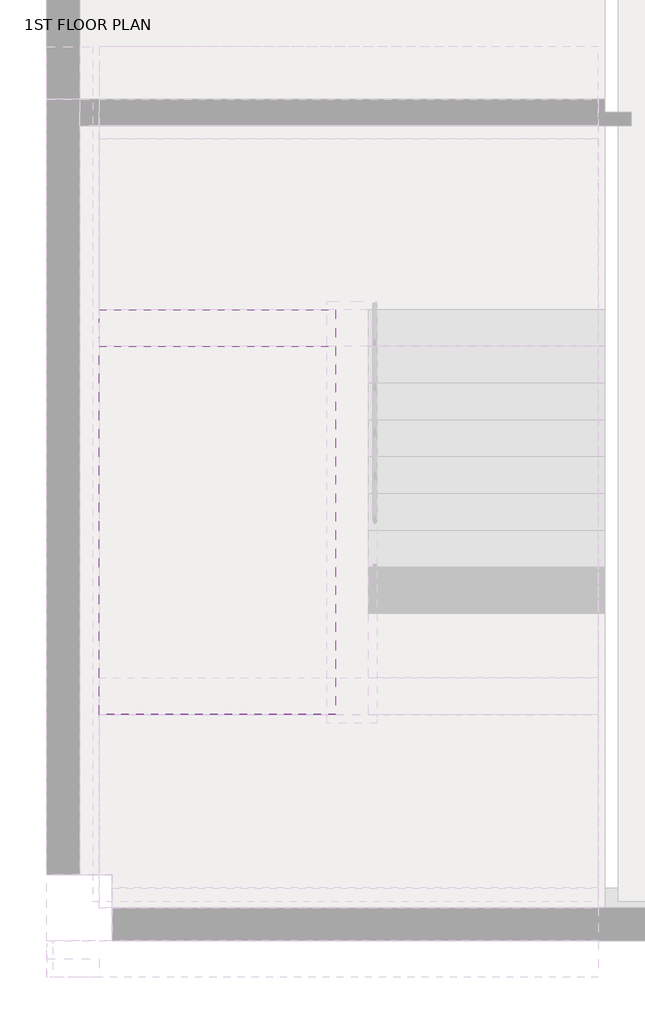
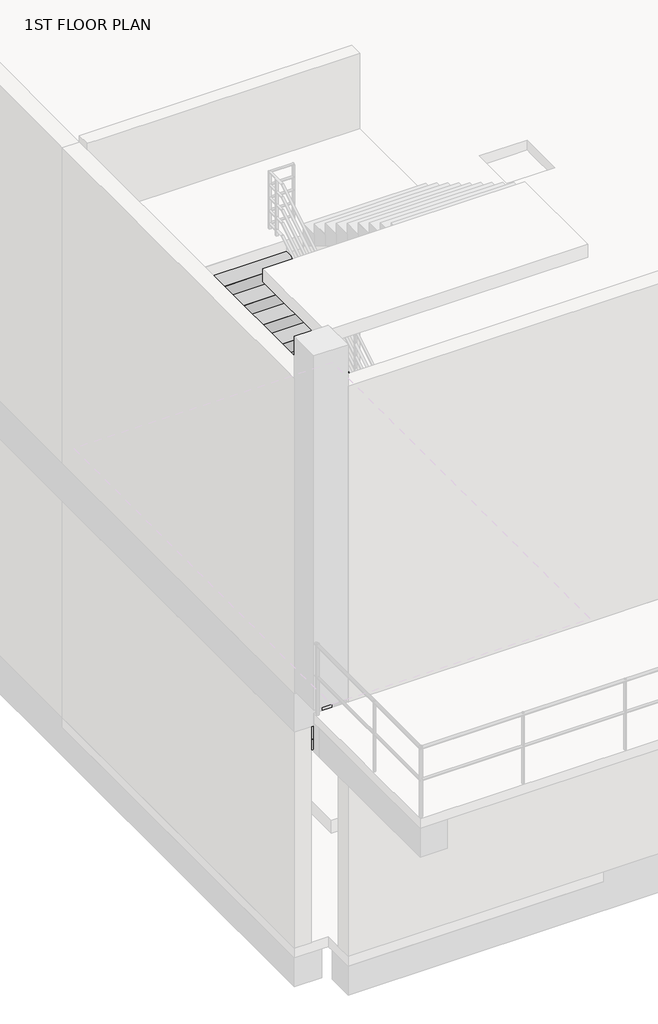
# One storey, part 6 of 9: 2 stair flights.
"""IFC4 building model written with IfcOpenShell, lengths in millimetres."""

from ifc_helpers import new_model, si_unit, frame, origin, place, context, project, spatial, polyline, outline, extrude, faceted_brep, element, save

model = new_model("IFC4")

# Units and contexts
model_context = context("Model", 3, world=origin())
ifc_project = project(units=[si_unit("LENGTHUNIT", "METRE", prefix="MILLI")], contexts=[model_context])

# Site, building, storey
site = spatial("IfcSite", under=ifc_project)
building = spatial("IfcBuilding", under=site)
storey = spatial("IfcBuildingStorey", under=building, Name="1ST FLOOR PLAN", Elevation=600.005241)

# Stair flights
placement = place(None, origin())
element("IfcStairFlight", 1, ObjectType="1mm 디딤판", at=placement, inside=storey, context=model_context, shape_type="SolidModel", body=[
    faceted_brep([(50.0, 22699.5208589, 2765.8781576), (50.0, 22419.5208589, 2765.8781576), (1850.0, 22419.5208589, 2765.8781576), (1850.0, 22699.5208589, 2765.8781576), (50.0, 22699.5208589, 2591.3160232), (50.0, 22419.5208589, 2424.6493565), (50.0, 22419.5208589, 2599.211491), (1850.0, 22419.5208589, 2424.6493565), (1850.0, 22699.5208589, 2591.3160232), (50.0, 22979.5208589, 2932.5448243), (50.0, 22699.5208589, 2932.5448243), (1850.0, 22699.5208589, 2932.5448243), (1850.0, 22979.5208589, 2932.5448243), (50.0, 22979.5208589, 2757.9826899), (1850.0, 22979.5208589, 2757.9826899), (50.0, 23259.5208589, 3099.211491), (50.0, 22979.5208589, 3099.211491), (1850.0, 22979.5208589, 3099.211491), (1850.0, 23259.5208589, 3099.211491), (50.0, 23259.5208589, 2924.6493565), (1850.0, 23259.5208589, 2924.6493565), (50.0, 23539.5208589, 3265.8781576), (50.0, 23259.5208589, 3265.8781576), (1850.0, 23259.5208589, 3265.8781576), (1850.0, 23539.5208589, 3265.8781576), (50.0, 23539.5208589, 3091.3160232), (1850.0, 23539.5208589, 3091.3160232), (50.0, 23819.5208589, 3432.5448243), (50.0, 23539.5208589, 3432.5448243), (1850.0, 23539.5208589, 3432.5448243), (1850.0, 23819.5208589, 3432.5448243), (50.0, 23819.5208589, 3257.9826899), (1850.0, 23819.5208589, 3257.9826899), (50.0, 24099.5208589, 3599.211491), (50.0, 23819.5208589, 3599.211491), (1850.0, 23819.5208589, 3599.211491), (1850.0, 24099.5208589, 3599.211491), (50.0, 24099.5208589, 3424.6493565), (1850.0, 24099.5208589, 3424.6493565), (50.0, 24379.5208589, 3765.8781576), (50.0, 24099.5208589, 3765.8781576), (1850.0, 24099.5208589, 3765.8781576), (1850.0, 24379.5208589, 3765.8781576), (50.0, 24379.5208589, 3591.3160232), (1850.0, 24379.5208589, 3591.3160232), (50.0, 24659.5208589, 3932.5448243), (50.0, 24379.5208589, 3932.5448243), (1850.0, 24379.5208589, 3932.5448243), (1850.0, 24659.5208589, 3932.5448243), (50.0, 24659.5208589, 3757.9826899), (1850.0, 24659.5208589, 3757.9826899), (50.0, 24939.5208589, 4099.211491), (50.0, 24659.5208589, 4099.211491), (1850.0, 24659.5208589, 4099.211491), (1850.0, 24939.5208589, 4099.211491), (50.0, 24939.5208589, 3924.6493565), (1850.0, 24939.5208589, 3924.6493565), (50.0, 25219.5208589, 4265.8781576), (50.0, 24939.5208589, 4265.8781576), (1850.0, 24939.5208589, 4265.8781576), (1850.0, 25219.5208589, 4265.8781576), (50.0, 25219.5208589, 4091.3160232), (1850.0, 25219.5208589, 4091.3160232), (50.0, 25499.5208589, 4432.5448243), (50.0, 25219.5208589, 4432.5448243), (1850.0, 25219.5208589, 4432.5448243), (1850.0, 25499.5208589, 4432.5448243), (50.0, 25499.5208589, 4257.9826899), (1850.0, 25499.5208589, 4257.9826899), (1850.0, 25499.5208589, 4399.211491)], [[[0, 1, 2, 3]], [[1, 0, 4, 5, 6]], [[2, 1, 6, 5, 7]], [[3, 2, 7, 8]], [[9, 10, 11, 12]], [[10, 9, 13, 4, 0]], [[11, 10, 0, 3]], [[12, 11, 3, 8, 14]], [[15, 16, 17, 18]], [[16, 15, 19, 13, 9]], [[17, 16, 9, 12]], [[18, 17, 12, 14, 20]], [[21, 22, 23, 24]], [[22, 21, 25, 19, 15]], [[23, 22, 15, 18]], [[24, 23, 18, 20, 26]], [[27, 28, 29, 30]], [[28, 27, 31, 25, 21]], [[29, 28, 21, 24]], [[30, 29, 24, 26, 32]], [[33, 34, 35, 36]], [[34, 33, 37, 31, 27]], [[35, 34, 27, 30]], [[36, 35, 30, 32, 38]], [[39, 40, 41, 42]], [[40, 39, 43, 37, 33]], [[41, 40, 33, 36]], [[42, 41, 36, 38, 44]], [[45, 46, 47, 48]], [[46, 45, 49, 43, 39]], [[47, 46, 39, 42]], [[48, 47, 42, 44, 50]], [[51, 52, 53, 54]], [[52, 51, 55, 49, 45]], [[53, 52, 45, 48]], [[54, 53, 48, 50, 56]], [[57, 58, 59, 60]], [[58, 57, 61, 55, 51]], [[59, 58, 51, 54]], [[60, 59, 54, 56, 62]], [[63, 64, 65, 66]], [[64, 63, 67, 61, 57]], [[65, 64, 57, 60]], [[66, 65, 60, 62, 68, 69]], [[63, 66, 69, 68, 67]], [[5, 4, 13, 19, 25, 31, 37, 43, 49, 55, 61, 67, 68, 62, 56, 50, 44, 38, 32, 26, 20, 14, 8, 7]]]),
    extrude(outline(polyline([(50.0, 22699.5208589), (1850.0, 22699.5208589), (1850.0, 22419.5208589), (50.0, 22419.5208589), (50.0, 22699.5208589)])), frame((0.0, 0.0, 2765.8781576), z_axis=(0.0, 0.0, 1.0), x_axis=(1.0, 0.0, 0.0)), (0.0, 0.0, 1.0), 0.79375),
    extrude(outline(polyline([(50.0, 22979.5208589), (1850.0, 22979.5208589), (1850.0, 22699.5208589), (50.0, 22699.5208589), (50.0, 22979.5208589)])), frame((0.0, 0.0, 2932.5448243), z_axis=(0.0, 0.0, 1.0), x_axis=(1.0, 0.0, 0.0)), (0.0, 0.0, 1.0), 0.79375),
    extrude(outline(polyline([(50.0, 23259.5208589), (1850.0, 23259.5208589), (1850.0, 22979.5208589), (50.0, 22979.5208589), (50.0, 23259.5208589)])), frame((0.0, 0.0, 3099.211491), z_axis=(0.0, 0.0, 1.0), x_axis=(1.0, 0.0, 0.0)), (0.0, 0.0, 1.0), 0.79375),
    extrude(outline(polyline([(50.0, 23539.5208589), (1850.0, 23539.5208589), (1850.0, 23259.5208589), (50.0, 23259.5208589), (50.0, 23539.5208589)])), frame((0.0, 0.0, 3265.8781576), z_axis=(0.0, 0.0, 1.0), x_axis=(1.0, 0.0, 0.0)), (0.0, 0.0, 1.0), 0.79375),
    extrude(outline(polyline([(50.0, 23819.5208589), (1850.0, 23819.5208589), (1850.0, 23539.5208589), (50.0, 23539.5208589), (50.0, 23819.5208589)])), frame((0.0, 0.0, 3432.5448243), z_axis=(0.0, 0.0, 1.0), x_axis=(1.0, 0.0, 0.0)), (0.0, 0.0, 1.0), 0.79375),
    extrude(outline(polyline([(50.0, 24099.5208589), (1850.0, 24099.5208589), (1850.0, 23819.5208589), (50.0, 23819.5208589), (50.0, 24099.5208589)])), frame((0.0, 0.0, 3599.211491), z_axis=(0.0, 0.0, 1.0), x_axis=(1.0, 0.0, 0.0)), (0.0, 0.0, 1.0), 0.79375),
    extrude(outline(polyline([(50.0, 24379.5208589), (1850.0, 24379.5208589), (1850.0, 24099.5208589), (50.0, 24099.5208589), (50.0, 24379.5208589)])), frame((0.0, 0.0, 3765.8781576), z_axis=(0.0, 0.0, 1.0), x_axis=(1.0, 0.0, 0.0)), (0.0, 0.0, 1.0), 0.79375),
    extrude(outline(polyline([(50.0, 24659.5208589), (1850.0, 24659.5208589), (1850.0, 24379.5208589), (50.0, 24379.5208589), (50.0, 24659.5208589)])), frame((0.0, 0.0, 3932.5448243), z_axis=(0.0, 0.0, 1.0), x_axis=(1.0, 0.0, 0.0)), (0.0, 0.0, 1.0), 0.79375),
    extrude(outline(polyline([(50.0, 24939.5208589), (1850.0, 24939.5208589), (1850.0, 24659.5208589), (50.0, 24659.5208589), (50.0, 24939.5208589)])), frame((0.0, 0.0, 4099.211491), z_axis=(0.0, 0.0, 1.0), x_axis=(1.0, 0.0, 0.0)), (0.0, 0.0, 1.0), 0.79375),
    extrude(outline(polyline([(50.0, 25219.5208589), (1850.0, 25219.5208589), (1850.0, 24939.5208589), (50.0, 24939.5208589), (50.0, 25219.5208589)])), frame((0.0, 0.0, 4265.8781576), z_axis=(0.0, 0.0, 1.0), x_axis=(1.0, 0.0, 0.0)), (0.0, 0.0, 1.0), 0.79375),
    extrude(outline(polyline([(50.0, 25499.5208589), (1850.0, 25499.5208589), (1850.0, 25219.5208589), (50.0, 25219.5208589), (50.0, 25499.5208589)])), frame((0.0, 0.0, 4432.5448243), z_axis=(0.0, 0.0, 1.0), x_axis=(1.0, 0.0, 0.0)), (0.0, 0.0, 1.0), 0.79375),
])
element("IfcStairFlight", 2, ObjectType="1mm 디딤판", at=placement, inside=storey, context=model_context, shape_type="SolidModel", body=[
    faceted_brep([(50.0, 22699.5208589, 6661.711491), (50.0, 22419.5208589, 6661.711491), (1850.0, 22419.5208589, 6661.711491), (1850.0, 22699.5208589, 6661.711491), (50.0, 22699.5208589, 6485.7058943), (50.0, 22419.5208589, 6313.8308943), (50.0, 22419.5208589, 6489.836491), (1850.0, 22419.5208589, 6313.8308943), (1850.0, 22699.5208589, 6485.7058943), (50.0, 22979.5208589, 6833.586491), (50.0, 22699.5208589, 6833.586491), (1850.0, 22699.5208589, 6833.586491), (1850.0, 22979.5208589, 6833.586491), (50.0, 22979.5208589, 6657.5808943), (1850.0, 22979.5208589, 6657.5808943), (50.0, 23259.5208589, 7005.461491), (50.0, 22979.5208589, 7005.461491), (1850.0, 22979.5208589, 7005.461491), (1850.0, 23259.5208589, 7005.461491), (50.0, 23259.5208589, 6829.4558943), (1850.0, 23259.5208589, 6829.4558943), (50.0, 23539.5208589, 7177.336491), (50.0, 23259.5208589, 7177.336491), (1850.0, 23259.5208589, 7177.336491), (1850.0, 23539.5208589, 7177.336491), (50.0, 23539.5208589, 7001.3308943), (1850.0, 23539.5208589, 7001.3308943), (50.0, 23819.5208589, 7349.211491), (50.0, 23539.5208589, 7349.211491), (1850.0, 23539.5208589, 7349.211491), (1850.0, 23819.5208589, 7349.211491), (50.0, 23819.5208589, 7173.2058943), (1850.0, 23819.5208589, 7173.2058943), (50.0, 24099.5208589, 7521.086491), (50.0, 23819.5208589, 7521.086491), (1850.0, 23819.5208589, 7521.086491), (1850.0, 24099.5208589, 7521.086491), (50.0, 24099.5208589, 7345.0808943), (1850.0, 24099.5208589, 7345.0808943), (50.0, 24379.5208589, 7692.961491), (50.0, 24099.5208589, 7692.961491), (1850.0, 24099.5208589, 7692.961491), (1850.0, 24379.5208589, 7692.961491), (50.0, 24379.5208589, 7516.9558943), (1850.0, 24379.5208589, 7516.9558943), (50.0, 24659.5208589, 7864.836491), (50.0, 24379.5208589, 7864.836491), (1850.0, 24379.5208589, 7864.836491), (1850.0, 24659.5208589, 7864.836491), (50.0, 24659.5208589, 7688.8308943), (1850.0, 24659.5208589, 7688.8308943), (50.0, 24939.5208589, 8036.711491), (50.0, 24659.5208589, 8036.711491), (1850.0, 24659.5208589, 8036.711491), (1850.0, 24939.5208589, 8036.711491), (50.0, 24939.5208589, 7860.7058943), (1850.0, 24939.5208589, 7860.7058943), (50.0, 25219.5208589, 8208.586491), (50.0, 24939.5208589, 8208.586491), (1850.0, 24939.5208589, 8208.586491), (1850.0, 25219.5208589, 8208.586491), (50.0, 25219.5208589, 8032.5808943), (1850.0, 25219.5208589, 8032.5808943), (1850.0, 25219.5208589, 8180.461491)], [[[0, 1, 2, 3]], [[1, 0, 4, 5, 6]], [[2, 1, 6, 5, 7]], [[3, 2, 7, 8]], [[9, 10, 11, 12]], [[10, 9, 13, 4, 0]], [[11, 10, 0, 3]], [[12, 11, 3, 8, 14]], [[15, 16, 17, 18]], [[16, 15, 19, 13, 9]], [[17, 16, 9, 12]], [[18, 17, 12, 14, 20]], [[21, 22, 23, 24]], [[22, 21, 25, 19, 15]], [[23, 22, 15, 18]], [[24, 23, 18, 20, 26]], [[27, 28, 29, 30]], [[28, 27, 31, 25, 21]], [[29, 28, 21, 24]], [[30, 29, 24, 26, 32]], [[33, 34, 35, 36]], [[34, 33, 37, 31, 27]], [[35, 34, 27, 30]], [[36, 35, 30, 32, 38]], [[39, 40, 41, 42]], [[40, 39, 43, 37, 33]], [[41, 40, 33, 36]], [[42, 41, 36, 38, 44]], [[45, 46, 47, 48]], [[46, 45, 49, 43, 39]], [[47, 46, 39, 42]], [[48, 47, 42, 44, 50]], [[51, 52, 53, 54]], [[52, 51, 55, 49, 45]], [[53, 52, 45, 48]], [[54, 53, 48, 50, 56]], [[57, 58, 59, 60]], [[58, 57, 61, 55, 51]], [[59, 58, 51, 54]], [[60, 59, 54, 56, 62, 63]], [[57, 60, 63, 62, 61]], [[5, 4, 13, 19, 25, 31, 37, 43, 49, 55, 61, 62, 56, 50, 44, 38, 32, 26, 20, 14, 8, 7]]]),
    extrude(outline(polyline([(50.0, 22699.5208589), (1850.0, 22699.5208589), (1850.0, 22419.5208589), (50.0, 22419.5208589), (50.0, 22699.5208589)])), frame((0.0, 0.0, 6661.711491), z_axis=(0.0, 0.0, 1.0), x_axis=(1.0, 0.0, 0.0)), (0.0, 0.0, 1.0), 0.79375),
    extrude(outline(polyline([(50.0, 22979.5208589), (1850.0, 22979.5208589), (1850.0, 22699.5208589), (50.0, 22699.5208589), (50.0, 22979.5208589)])), frame((0.0, 0.0, 6833.586491), z_axis=(0.0, 0.0, 1.0), x_axis=(1.0, 0.0, 0.0)), (0.0, 0.0, 1.0), 0.79375),
    extrude(outline(polyline([(50.0, 23259.5208589), (1850.0, 23259.5208589), (1850.0, 22979.5208589), (50.0, 22979.5208589), (50.0, 23259.5208589)])), frame((0.0, 0.0, 7005.461491), z_axis=(0.0, 0.0, 1.0), x_axis=(1.0, 0.0, 0.0)), (0.0, 0.0, 1.0), 0.79375),
    extrude(outline(polyline([(50.0, 23539.5208589), (1850.0, 23539.5208589), (1850.0, 23259.5208589), (50.0, 23259.5208589), (50.0, 23539.5208589)])), frame((0.0, 0.0, 7177.336491), z_axis=(0.0, 0.0, 1.0), x_axis=(1.0, 0.0, 0.0)), (0.0, 0.0, 1.0), 0.79375),
    extrude(outline(polyline([(50.0, 23819.5208589), (1850.0, 23819.5208589), (1850.0, 23539.5208589), (50.0, 23539.5208589), (50.0, 23819.5208589)])), frame((0.0, 0.0, 7349.211491), z_axis=(0.0, 0.0, 1.0), x_axis=(1.0, 0.0, 0.0)), (0.0, 0.0, 1.0), 0.79375),
    extrude(outline(polyline([(50.0, 24099.5208589), (1850.0, 24099.5208589), (1850.0, 23819.5208589), (50.0, 23819.5208589), (50.0, 24099.5208589)])), frame((0.0, 0.0, 7521.086491), z_axis=(0.0, 0.0, 1.0), x_axis=(1.0, 0.0, 0.0)), (0.0, 0.0, 1.0), 0.79375),
    extrude(outline(polyline([(50.0, 24379.5208589), (1850.0, 24379.5208589), (1850.0, 24099.5208589), (50.0, 24099.5208589), (50.0, 24379.5208589)])), frame((0.0, 0.0, 7692.961491), z_axis=(0.0, 0.0, 1.0), x_axis=(1.0, 0.0, 0.0)), (0.0, 0.0, 1.0), 0.79375),
    extrude(outline(polyline([(50.0, 24659.5208589), (1850.0, 24659.5208589), (1850.0, 24379.5208589), (50.0, 24379.5208589), (50.0, 24659.5208589)])), frame((0.0, 0.0, 7864.836491), z_axis=(0.0, 0.0, 1.0), x_axis=(1.0, 0.0, 0.0)), (0.0, 0.0, 1.0), 0.79375),
    extrude(outline(polyline([(50.0, 24939.5208589), (1850.0, 24939.5208589), (1850.0, 24659.5208589), (50.0, 24659.5208589), (50.0, 24939.5208589)])), frame((0.0, 0.0, 8036.711491), z_axis=(0.0, 0.0, 1.0), x_axis=(1.0, 0.0, 0.0)), (0.0, 0.0, 1.0), 0.79375),
    extrude(outline(polyline([(50.0, 25219.5208589), (1850.0, 25219.5208589), (1850.0, 24939.5208589), (50.0, 24939.5208589), (50.0, 25219.5208589)])), frame((0.0, 0.0, 8208.586491), z_axis=(0.0, 0.0, 1.0), x_axis=(1.0, 0.0, 0.0)), (0.0, 0.0, 1.0), 0.79375),
])

save(model, "model.ifc")

# Revit data of these elements
# Elements 1, 2 (IfcStairFlight, "1mm 디딤판")
#   Phase Created = New Construction
#   Materials on its faces: "A03AD032-00007_Structural Concrete_25MPa-30MPa"
# Materials
#   "A03AD032-00007_Structural Concrete_25MPa-30MPa": class "Concrete", colour RGB 176 176 176, transparency 0, Keynote = "09910.A1", Description = "ACRYLIC EMULSION PAINT ON\nFAIR FACED CONC.", W00) Work Master Code = "A03AD032-00007", W01) Work Master_Lv1 = "Concrete Work", W02) Work Master_Lv2 = "Superstructure Work", W03) Work Master_Spec.1 = "Structural Concrete", W04) Work Master_Spec.2 = "Cement Type-1", W05) Work Master_Spec.3 = "25MPa < F'c (Cylinder Strength) ≤ 30MPa", Cost = 0
# Room at (20464.261, 36395.885) mm, phase "New Construction", upper level "1ST FLOOR PLAN", upper offset 3800 mm, lower offset 0 mm
#   Comments = ""
#   Base Finish = "EPOXY PAINT"
#   Ceiling Finish = "WATER EMULSOIN PAINT"
#   Wall Finish = "WATER EMULSION PAINT"
#   Floor Finish = "EPOXY PAINT ON STEEL TROWEL FINISH"
#   Number = "101"
#   Name = "CABLE ROOM"
#   S01) Room Name = ""
#   S02) Room Number(Project) = ""
#   FLOOR LEVEL = "1ST FLOOR PLAN"
# Room at (38671.941, 34306.947) mm, phase "New Construction", upper level "1ST FLOOR PLAN", upper offset 3800 mm, lower offset 0 mm
#   Comments = ""
#   Base Finish = "-"
#   Ceiling Finish = "ACID/ALKALINE RESISTANT PAINT"
#   Wall Finish = "ACID/ALKALINE RESISTANT PAINT"
#   Floor Finish = "ACID/ALKALINE RESISTANT PAINT ON STEEL TROWEL FINISH"
#   Number = "102"
#   Name = "BATTERY ROOM"
#   S01) Room Name = ""
#   S02) Room Number(Project) = ""
# Room at (5838.486, 24198.591) mm, phase "New Construction", upper level "1ST FLOOR PLAN", upper offset 3000 mm, lower offset 0 mm
#   Comments = ""
#   Base Finish = "VINYL TILE"
#   Ceiling Finish = "ACOUSTIC TILED CEILING(M-BAR)"
#   Wall Finish = "WATER EMULSION PAINT"
#   Floor Finish = "VINYL TILE W/MORTAR BOND COAT OR ADHESIVE"
#   Number = "103"
#   Name = "ROBBY"
#   S01) Room Name = ""
#   S02) Room Number(Project) = ""
# Room at (20756.85, 25498.466) mm, phase "New Construction", upper level "2ND FLOOR PLAN", upper offset 5300 mm, lower offset 0 mm
#   Comments = ""
#   Base Finish = "EPOXY PAINT"
#   Ceiling Finish = "WATER EMULSOIN PAINT"
#   Wall Finish = "WATER EMULSION PAINT"
#   Floor Finish = "EPOXY PAINT ON CEMENT MORTAR"
#   Number = "201"
#   Name = "ELECTRICAL ROOM"
#   S01) Room Name = ""
#   S02) Room Number(Project) = ""
#   FLOOR LEVEL = "2ST FLOOR PLAN"
# Room at (2015.811, 21738.481) mm, phase "New Construction", upper level "1ST FLOOR PLAN", upper offset 2000 mm, lower offset 0 mm
#   Comments = ""
#   Base Finish = "VINYL TILE"
#   Ceiling Finish = "WATER EMULSOIN PAINT"
#   Wall Finish = "WATER EMULSION PAINT"
#   Floor Finish = "VINYL TILE W/MORTAR BOND COAT OR ADHESIVE"
#   Number = "104"
#   Name = "STAIR-1"
#   S01) Room Name = ""
#   S02) Room Number(Project) = ""
# Room at (12026.665, 34535.731) mm, phase "New Construction", upper level "2ND FLOOR PLAN", upper offset 5300 mm, lower offset 0 mm
#   Comments = ""
#   Base Finish = "EPOXY PAINT"
#   Ceiling Finish = "WATER EMULSOIN PAINT"
#   Wall Finish = "WATER EMULSION PAINT"
#   Floor Finish = "EPOXY PAINT ON CEMENT MORTAR"
#   Number = "202"
#   Name = "ELECTRICAL ROOM-2"
#   S01) Room Name = ""
#   S02) Room Number(Project) = ""
# Room at (37132.151, 34229.96) mm, phase "New Construction", upper level "2ND FLOOR PLAN", upper offset 5300 mm, lower offset 0 mm
#   Comments = ""
#   Base Finish = "EPOXY PAINT"
#   Ceiling Finish = "WATER EMULSOIN PAINT"
#   Wall Finish = "WATER EMULSION PAINT"
#   Floor Finish = "EPOXY PAINT ON CEMENT MORTAR"
#   Number = "203"
#   Name = "ELECTRICAL ROOM(GIS)"
#   S01) Room Name = ""
#   S02) Room Number(Project) = ""
# Room at (5905.828, 24140.385) mm, phase "New Construction", upper level "2ND FLOOR PLAN", upper offset 3000 mm, lower offset 0 mm
#   Comments = ""
#   Base Finish = "VINYL TILE"
#   Ceiling Finish = "ACOUSTIC TILED CEILING(M-BAR)"
#   Wall Finish = "WATER EMULSION PAINT"
#   Floor Finish = "VINYL TILE W/MORTAR BOND COAT OR ADHESIVE"
#   Number = "204"
#   Name = "ROBBY"
#   S01) Room Name = ""
#   S02) Room Number(Project) = ""
# Room at (2027.324, 21779.624) mm, phase "New Construction", upper level "2ND FLOOR PLAN", upper offset 2000 mm, lower offset 0 mm
#   Comments = ""
#   Base Finish = "VINYL TILE"
#   Ceiling Finish = "WATER EMULSOIN PAINT"
#   Wall Finish = "WATER EMULSION PAINT"
#   Floor Finish = "VINYL TILE W/MORTAR BOND COAT OR ADHESIVE"
#   Number = "205"
#   Name = "STAIR-1"
#   S01) Room Name = ""
#   S02) Room Number(Project) = ""
